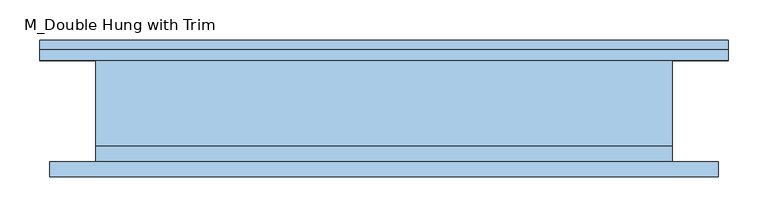
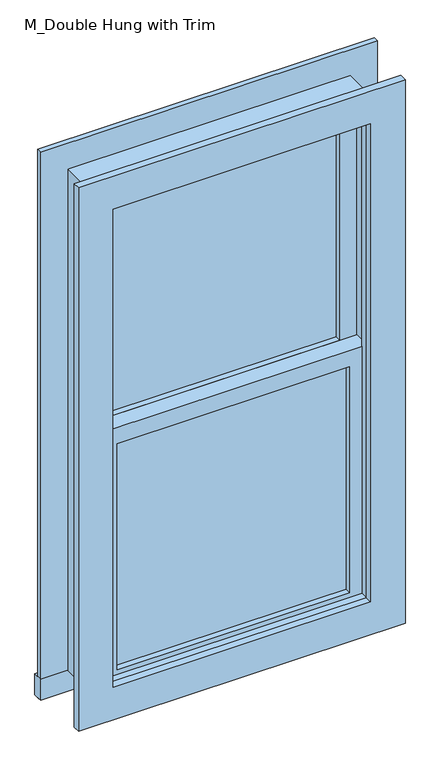
"""IFC4 building model written with IfcOpenShell, lengths in millimetres: window geometry, M_Double Hung with Trim."""

from ifc_helpers import new_model, si_unit, frame, origin, place, context, project, spatial, polyline, outline, extrude, source, transform, mapped, element, save


def m_double_hung_with_trim_a199e264(model_context):
    return source(origin(), model_context, "Body", "SweptSolid", [
        extrude(outline(polyline([(-298.45, -15.825), (298.45, -15.825), (298.45, -28.525), (-298.45, -28.525), (-298.45, -15.825)])), frame((0.0, 0.0, 628.65), z_axis=(0.0, 0.0, 1.0), x_axis=(1.0, 0.0, 0.0)), (0.0, 0.0, 1.0), 612.775),
        extrude(outline(polyline([(1285.875, -342.9), (584.2, -342.9), (584.2, 342.9), (1285.875, 342.9), (1285.875, -342.9)]), holes=[polyline([(1241.425, -298.45), (1241.425, 298.45), (628.65, 298.45), (628.65, -298.45), (1241.425, -298.45)])]), frame((0.0, -44.4, 0.0), z_axis=(0.0, 1.0, 0.0), x_axis=(0.0, 0.0, 1.0)), (0.0, 0.0, 1.0), 44.45),
        extrude(outline(polyline([(-431.9, 89.2), (431.9, 89.2), (431.9, 63.5), (-431.9, 63.5), (-431.9, 89.2)])), frame((0.0, 0.0, 526.95), z_axis=(0.0, 0.0, 1.0), x_axis=(1.0, 0.0, 0.0)), (0.0, 0.0, 1.0), 57.25),
        extrude(outline(polyline([(2013.05, -431.9), (526.95, -431.9), (526.95, 431.9), (2013.05, 431.9), (2013.05, -431.9)]), holes=[polyline([(1924.05, -342.9), (1924.05, 342.9), (584.2, 342.9), (584.2, -342.9), (1924.05, -342.9)])]), frame((0.0, 63.5, 0.0), z_axis=(0.0, 1.0, 0.0), x_axis=(0.0, 0.0, 1.0)), (0.0, 0.0, 1.0), 13.0),
        extrude(outline(polyline([(2000.35, 419.2), (2000.35, -419.2), (526.95, -419.2), (526.95, 419.2), (2000.35, 419.2)]), holes=[polyline([(1911.35, 330.2), (615.95, 330.2), (615.95, -330.2), (1911.35, -330.2), (1911.35, 330.2)])]), frame((0.0, -82.5, 0.0), z_axis=(0.0, 1.0, 0.0), x_axis=(0.0, 0.0, 1.0)), (0.0, 0.0, 1.0), 19.0),
        extrude(outline(polyline([(298.45, 15.925), (-298.45, 15.925), (-298.45, 28.625), (298.45, 28.625), (298.45, 15.925)])), frame((0.0, 0.0, 1285.875), z_axis=(0.0, 0.0, 1.0), x_axis=(1.0, 0.0, 0.0)), (0.0, 0.0, 1.0), 593.725),
        extrude(outline(polyline([(1924.05, -342.9), (1241.425, -342.9), (1241.425, 342.9), (1924.05, 342.9), (1924.05, -342.9)]), holes=[polyline([(1879.6, -298.45), (1879.6, 298.45), (1285.875, 298.45), (1285.875, -298.45), (1879.6, -298.45)])]), frame((0.0, 0.05, 0.0), z_axis=(0.0, 1.0, 0.0), x_axis=(0.0, 0.0, 1.0)), (0.0, 0.0, 1.0), 44.45),
        extrude(outline(polyline([(1943.1, -361.95), (584.2, -361.95), (584.2, 361.95), (1943.1, 361.95), (1943.1, -361.95)]), holes=[polyline([(1911.35, -330.2), (1911.35, 330.2), (615.95, 330.2), (615.95, -330.2), (1911.35, -330.2)])]), frame((0.0, -63.5, 0.0), z_axis=(0.0, 1.0, 0.0), x_axis=(0.0, 0.0, 1.0)), (0.0, 0.0, 1.0), 19.1),
        extrude(outline(polyline([(1943.1, 361.95), (1943.1, -361.95), (584.2, -361.95), (584.2, 361.95), (1943.1, 361.95)]), holes=[polyline([(1924.05, 342.9), (603.25, 342.9), (603.25, -342.9), (1924.05, -342.9), (1924.05, 342.9)])]), frame((0.0, -44.4, 0.0), z_axis=(0.0, 1.0, 0.0), x_axis=(0.0, 0.0, 1.0)), (0.0, 0.0, 1.0), 107.9),
    ])


if __name__ == "__main__":
    model = new_model("IFC4")
    model_context = context("Model", 3, world=origin())
    ifc_project = project(units=[si_unit("LENGTHUNIT", "METRE", prefix="MILLI")], contexts=[model_context])
    site = spatial("IfcSite", under=ifc_project)
    building = spatial("IfcBuilding", under=site)
    placement = place(None, origin())
    m_double_hung_with_trim_shape = m_double_hung_with_trim_a199e264(model_context)
    element("IfcWindow", 1, ObjectType="M_Double Hung with Trim : 57\" x 54\" @ 23\" b", at=placement, inside=building, context=model_context, shape_type="MappedRepresentation", body=[
        mapped(m_double_hung_with_trim_shape, transform((0.0, 0.0, 0.0), x_axis=(1.0, 0.0, 0.0), y_axis=(0.0, 1.0, 0.0), z_axis=(0.0, 0.0, 1.0))),
    ])
    save(model, "model.ifc")

# Revit data of these elements
# Type "M_Double Hung with Trim : 57\" x 54\" @ 23\" b"
#   Type Mark = "63"
#   Construction Type Id = "GSP4R"
#   Analytic Construction = "1/8 in Pilkington single glazing"
#   Visual Light Transmittance = 0.9
#   Thermal Resistance (R) = 0.271106 (m²·K)/W
#   Solar Heat Gain Coefficient = 0.78
#   Heat Transfer Coefficient (U) = 3.6886 W/(m²·K)
#   Height = 4' - 5 1/2"
#   Default Sill Height = 1' - 11"
#   Trim Projection - Ext. = 0' - 0.51181"
#   Trim Projection - Int. = 0' - 0.74803"
#   Trim Width - Exterior = 0' - 3.50394"
#   Trim Width - Interior = 0' - 3.50394"
#   Width = 2' - 4 1/2"
#   Window Inset = 0' - 0.74803"
#   Glass Pane Material = EXISTING WINDOW
#   Sash = Trim
#   Trim Exterior Material = Trim
#   Trim Interior Material = Trim
#   Wall Closure = (empty or 0)
# Element 1 (IfcWindow, "M_Double Hung with Trim : 57\" x 54\" @ 23\" b")
#   Materials on its faces: "Trim", "EXISTING WINDOW"
# Materials
#   "EXISTING WINDOW": class "Glass", colour RGB 218 227 224, transparency 0.85, Description = "Soda Lime Glass", Cost = 0
#   "Trim": class "Wood", colour RGB 250 251 245, transparency 0, Cost = 0
